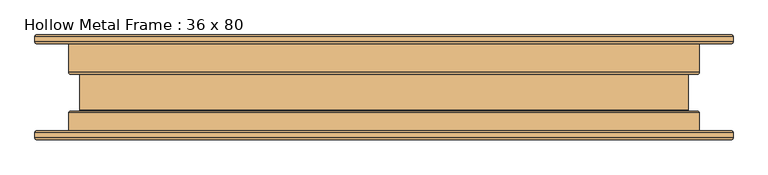
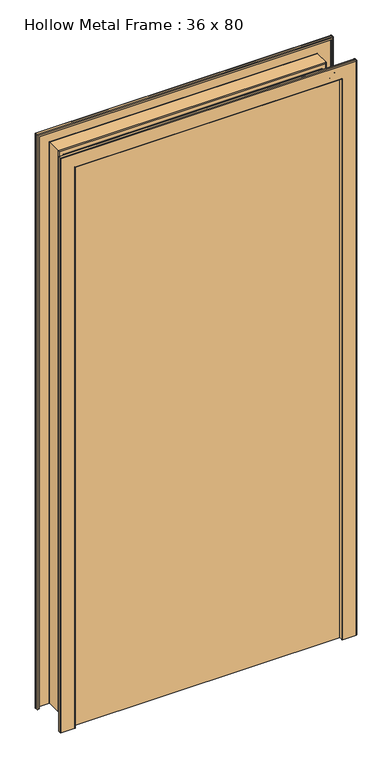
"""IFC4 building model written with IfcOpenShell, lengths in millimetres: door geometry, Hollow Metal Frame : 36 x 80."""

from ifc_helpers import new_model, si_unit, frame, origin, origin_with_axes, place, context, project, spatial, polyline, circle_curve, ellipse_curve, outline, extrude, source, transform, mapped, element, save
from ifc_brep_helpers import plane_surface, cylinder_surface, revolved_surface, advanced_brep


def hollow_metal_frame_36_x_80_d56a384a(model_context):
    return source(origin(), model_context, "Body", "SolidModel", [
        advanced_brep(
        [(-505.42825, 63.5635, 0.0), (-508.0, 66.13525, 0.0), (-508.0, 73.66, 0.0), (-505.42825, 76.23175, 0.0), (-459.77175, 76.23175, 0.0), (-457.2, 73.66, 0.0), (-457.2, 21.68525, 0.0), (-456.184, 20.66925, 0.0), (-443.89675, 20.66925, 0.0), (-441.325, 18.0975, 0.0), (-441.325, -33.6931, 0.0), (-443.89675, -36.26485, 0.0), (-456.184, -36.26485, 0.0), (-457.2, -37.28085, 0.0), (-457.2, -73.5965, 0.0), (-459.77175, -76.16825, 0.0), (-505.42825, -76.16825, 0.0), (-508.0, -73.5965, 0.0), (-508.0, -66.07175, 0.0), (-505.42825, -63.5, 0.0), (-500.0625, -63.5, 0.0), (-500.0625, -65.05575, 0.0), (-505.42825, -65.05575, 0.0), (-506.44425, -66.07175, 0.0), (-506.44425, -73.5965, 0.0), (-505.42825, -74.6125, 0.0), (-459.77175, -74.6125, 0.0), (-458.75575, -73.5965, 0.0), (-458.75575, -37.28085, 0.0), (-456.184, -34.7091, 0.0), (-443.89675, -34.7091, 0.0), (-442.88075, -33.6931, 0.0), (-442.88075, 18.0975, 0.0), (-443.89675, 19.1135, 0.0), (-456.184, 19.1135, 0.0), (-458.75575, 21.68525, 0.0), (-458.75575, 73.66, 0.0), (-459.77175, 74.676, 0.0), (-505.42825, 74.676, 0.0), (-506.44425, 73.66, 0.0), (-506.44425, 66.13525, 0.0), (-505.42825, 65.11925, 0.0), (-500.0625, 65.11925, 0.0), (-500.0625, 63.5635, 0.0), (-505.42825, 63.5635, 2080.2282501), (-508.0, 66.13525, 2082.8000001), (-508.0, 73.66, 2082.8000001), (-505.42825, 76.23175, 2080.2282501), (505.42825, 76.23175, 2080.2282501), (505.42825, 76.23175, 0.0), (459.77175, 76.23175, 0.0), (459.77175, 76.23175, 2034.5717501), (-459.77175, 76.23175, 2034.5717501), (-457.2, 73.66, 2032.0000001), (-457.2, 21.68525, 2032.0000001), (-456.184, 20.66925, 2030.9840001), (456.184, 20.66925, 2030.9840001), (456.184, 20.66925, 0.0), (443.89675, 20.66925, 0.0), (443.89675, 20.66925, 2018.6967501), (-443.89675, 20.66925, 2018.6967501), (-441.325, 18.0975, 2016.1250001), (-441.325, -33.6931, 2016.1250001), (-443.89675, -36.26485, 2018.6967501), (443.89675, -36.26485, 2018.6967501), (443.89675, -36.26485, 0.0), (456.184, -36.26485, 0.0), (456.184, -36.26485, 2030.9840001), (-456.184, -36.26485, 2030.9840001), (-457.2, -37.28085, 2032.0000001), (-457.2, -73.5965, 2032.0000001), (-459.77175, -76.16825, 2034.5717501), (459.77175, -76.16825, 2034.5717501), (459.77175, -76.16825, 0.0), (505.42825, -76.16825, 0.0), (505.42825, -76.16825, 2080.2282501), (-505.42825, -76.16825, 2080.2282501), (-508.0, -73.5965, 2082.8000001), (-508.0, -66.07175, 2082.8000001), (-505.42825, -63.5, 2080.2282501), (505.42825, -63.5, 2080.2282501), (505.42825, -63.5, 0.0), (500.0625, -63.5, 0.0), (500.0625, -63.5, 2074.8625001), (-500.0625, -63.5, 2074.8625001), (-500.0625, -65.05575, 2074.8625001), (500.0625, -65.05575, 2074.8625001), (500.0625, -65.05575, 0.0), (505.42825, -65.05575, 0.0), (505.42825, -65.05575, 2080.2282501), (-505.42825, -65.05575, 2080.2282501), (-506.44425, -66.07175, 2081.2442501), (-506.44425, -73.5965, 2081.2442501), (-505.42825, -74.6125, 2080.2282501), (505.42825, -74.6125, 2080.2282501), (505.42825, -74.6125, 0.0), (459.77175, -74.6125, 0.0), (459.77175, -74.6125, 2034.5717501), (-459.77175, -74.6125, 2034.5717501), (-458.75575, -73.5965, 2033.5557501), (-458.75575, -37.28085, 2033.5557501), (-456.184, -34.7091, 2030.9840001), (456.184, -34.7091, 2030.9840001), (456.184, -34.7091, 0.0), (443.89675, -34.7091, 0.0), (443.89675, -34.7091, 2018.6967501), (-443.89675, -34.7091, 2018.6967501), (-442.88075, -33.6931, 2017.6807501), (-442.88075, 18.0975, 2017.6807501), (-443.89675, 19.1135, 2018.6967501), (443.89675, 19.1135, 2018.6967501), (443.89675, 19.1135, 0.0), (456.184, 19.1135, 0.0), (456.184, 19.1135, 2030.9840001), (-456.184, 19.1135, 2030.9840001), (-458.75575, 21.68525, 2033.5557501), (-458.75575, 73.66, 2033.5557501), (-459.77175, 74.676, 2034.5717501), (459.77175, 74.676, 2034.5717501), (459.77175, 74.676, 0.0), (505.42825, 74.676, 0.0), (505.42825, 74.676, 2080.2282501), (-505.42825, 74.676, 2080.2282501), (-506.44425, 73.66, 2081.2442501), (-506.44425, 66.13525, 2081.2442501), (-505.42825, 65.11925, 2080.2282501), (505.42825, 65.11925, 2080.2282501), (505.42825, 65.11925, 0.0), (500.0625, 65.11925, 0.0), (500.0625, 65.11925, 2074.8625001), (-500.0625, 65.11925, 2074.8625001), (-500.0625, 63.5635, 2074.8625001), (500.0625, 63.5635, 2074.8625001), (500.0625, 63.5635, 0.0), (505.42825, 63.5635, 0.0), (505.42825, 63.5635, 2080.2282501), (508.0, 66.13525, 2082.8000001), (508.0, 73.66, 2082.8000001), (457.2, 73.66, 2032.0000001), (457.2, 21.68525, 2032.0000001), (441.325, 18.0975, 2016.1250001), (441.325, -33.6931, 2016.1250001), (457.2, -37.28085, 2032.0000001), (457.2, -73.5965, 2032.0000001), (508.0, -73.5965, 2082.8000001), (508.0, -66.07175, 2082.8000001), (506.44425, -66.07175, 2081.2442501), (506.44425, -73.5965, 2081.2442501), (458.75575, -73.5965, 2033.5557501), (458.75575, -37.28085, 2033.5557501), (442.88075, -33.6931, 2017.6807501), (442.88075, 18.0975, 2017.6807501), (458.75575, 21.68525, 2033.5557501), (458.75575, 73.66, 2033.5557501), (506.44425, 73.66, 2081.2442501), (506.44425, 66.13525, 2081.2442501), (506.44425, 66.13525, 0.0), (506.44425, 73.66, 0.0), (458.75575, 73.66, 0.0), (458.75575, 21.68525, 0.0), (442.88075, 18.0975, 0.0), (442.88075, -33.6931, 0.0), (458.75575, -37.28085, 0.0), (458.75575, -73.5965, 0.0), (506.44425, -73.5965, 0.0), (506.44425, -66.07175, 0.0), (508.0, -66.07175, 0.0), (508.0, -73.5965, 0.0), (457.2, -73.5965, 0.0), (457.2, -37.28085, 0.0), (441.325, -33.6931, 0.0), (441.325, 18.0975, 0.0), (457.2, 21.68525, 0.0), (457.2, 73.66, 0.0), (508.0, 73.66, 0.0), (508.0, 66.13525, 0.0)],
        [
            (0, 1, circle_curve(frame((-505.42825, 66.13525, 0.0), z_axis=(0.0, 0.0, -1.0), x_axis=(0.0, -1.0, 0.0)), 2.57175)),
            (1, 2),
            (2, 3, circle_curve(frame((-505.42825, 73.66, 0.0), z_axis=(0.0, 0.0, -1.0), x_axis=(0.0, -1.0, 0.0)), 2.57175)),
            (3, 4),
            (4, 5, circle_curve(frame((-459.77175, 73.66, 0.0), z_axis=(0.0, 0.0, -1.0), x_axis=(0.0, -1.0, 0.0)), 2.57175)),
            (5, 6),
            (6, 7, circle_curve(frame((-456.184, 21.68525, 0.0), z_axis=(0.0, 0.0, 1.0), x_axis=(0.0, -1.0, 0.0)), 1.016)),
            (7, 8),
            (8, 9, circle_curve(frame((-443.89675, 18.0975, 0.0), z_axis=(0.0, 0.0, -1.0), x_axis=(0.0, -1.0, 0.0)), 2.57175)),
            (9, 10),
            (10, 11, circle_curve(frame((-443.89675, -33.6931, 0.0), z_axis=(0.0, 0.0, -1.0), x_axis=(0.0, -1.0, 0.0)), 2.57175)),
            (11, 12),
            (12, 13, circle_curve(frame((-456.184, -37.28085, 0.0), z_axis=(0.0, 0.0, 1.0), x_axis=(0.0, -1.0, 0.0)), 1.016)),
            (13, 14),
            (14, 15, circle_curve(frame((-459.77175, -73.5965, 0.0), z_axis=(0.0, 0.0, -1.0), x_axis=(0.0, -1.0, 0.0)), 2.57175)),
            (15, 16),
            (16, 17, circle_curve(frame((-505.42825, -73.5965, 0.0), z_axis=(0.0, 0.0, -1.0), x_axis=(0.0, -1.0, 0.0)), 2.57175)),
            (17, 18),
            (18, 19, circle_curve(frame((-505.42825, -66.07175, 0.0), z_axis=(0.0, 0.0, -1.0), x_axis=(0.0, -1.0, 0.0)), 2.57175)),
            (19, 20),
            (20, 21),
            (21, 22),
            (22, 23, circle_curve(frame((-505.42825, -66.07175, 0.0), z_axis=(0.0, 0.0, 1.0), x_axis=(0.0, -1.0, 0.0)), 1.016)),
            (23, 24),
            (24, 25, circle_curve(frame((-505.42825, -73.5965, 0.0), z_axis=(0.0, 0.0, 1.0), x_axis=(0.0, -1.0, 0.0)), 1.016)),
            (25, 26),
            (26, 27, circle_curve(frame((-459.77175, -73.5965, 0.0), z_axis=(0.0, 0.0, 1.0), x_axis=(0.0, -1.0, 0.0)), 1.016)),
            (27, 28),
            (28, 29, circle_curve(frame((-456.184, -37.28085, 0.0), z_axis=(0.0, 0.0, -1.0), x_axis=(0.0, -1.0, 0.0)), 2.57175)),
            (29, 30),
            (30, 31, circle_curve(frame((-443.89675, -33.6931, 0.0), z_axis=(0.0, 0.0, 1.0), x_axis=(0.0, -1.0, 0.0)), 1.016)),
            (31, 32),
            (32, 33, circle_curve(frame((-443.89675, 18.0975, 0.0), z_axis=(0.0, 0.0, 1.0), x_axis=(0.0, -1.0, 0.0)), 1.016)),
            (33, 34),
            (34, 35, circle_curve(frame((-456.184, 21.68525, 0.0), z_axis=(0.0, 0.0, -1.0), x_axis=(0.0, -1.0, 0.0)), 2.57175)),
            (35, 36),
            (36, 37, circle_curve(frame((-459.77175, 73.66, 0.0), z_axis=(0.0, 0.0, 1.0), x_axis=(0.0, -1.0, 0.0)), 1.016)),
            (37, 38),
            (38, 39, circle_curve(frame((-505.42825, 73.66, 0.0), z_axis=(0.0, 0.0, 1.0), x_axis=(0.0, -1.0, 0.0)), 1.016)),
            (39, 40),
            (40, 41, circle_curve(frame((-505.42825, 66.13525, 0.0), z_axis=(0.0, 0.0, 1.0), x_axis=(0.0, -1.0, 0.0)), 1.016)),
            (41, 42),
            (42, 43),
            (43, 0),
            (0, 44),
            (44, 45, ellipse_curve(frame((-505.42825, 66.13525, 2080.2282501), z_axis=(-0.7071067811865475, 0.0, -0.7071067811865475), x_axis=(0.7071067811865474, 0.0, -0.7071067811865476)), 3.6370037, 2.57175)),
            (45, 1),
            (45, 46),
            (46, 2),
            (46, 47, ellipse_curve(frame((-505.42825, 73.66, 2080.2282501), z_axis=(-0.7071067811865475, 0.0, -0.7071067811865475), x_axis=(0.7071067811865474, 0.0, -0.7071067811865476)), 3.6370037, 2.57175)),
            (47, 3),
            (47, 48),
            (48, 49),
            (49, 50),
            (50, 51),
            (51, 52),
            (52, 4),
            (52, 53, ellipse_curve(frame((-459.77175, 73.66, 2034.5717501), z_axis=(-0.7071067811865475, 0.0, -0.7071067811865475), x_axis=(0.7071067811865474, 0.0, -0.7071067811865476)), 3.6370037, 2.57175)),
            (53, 5),
            (53, 54),
            (54, 6),
            (54, 55, ellipse_curve(frame((-456.184, 21.68525, 2030.9840001), z_axis=(0.7071067811865475, 0.0, 0.7071067811865475), x_axis=(-0.7071067811865474, 0.0, 0.7071067811865476)), 1.436841, 1.016)),
            (55, 7),
            (55, 56),
            (56, 57),
            (57, 58),
            (58, 59),
            (59, 60),
            (60, 8),
            (60, 61, ellipse_curve(frame((-443.89675, 18.0975, 2018.6967501), z_axis=(-0.7071067811865475, 0.0, -0.7071067811865475), x_axis=(0.7071067811865474, 0.0, -0.7071067811865476)), 3.6370037, 2.57175)),
            (61, 9),
            (61, 62),
            (62, 10),
            (62, 63, ellipse_curve(frame((-443.89675, -33.6931, 2018.6967501), z_axis=(-0.7071067811865475, 0.0, -0.7071067811865475), x_axis=(0.7071067811865474, 0.0, -0.7071067811865476)), 3.6370037, 2.57175)),
            (63, 11),
            (63, 64),
            (64, 65),
            (65, 66),
            (66, 67),
            (67, 68),
            (68, 12),
            (68, 69, ellipse_curve(frame((-456.184, -37.28085, 2030.9840001), z_axis=(0.7071067811865475, 0.0, 0.7071067811865475), x_axis=(-0.7071067811865474, 0.0, 0.7071067811865476)), 1.436841, 1.016)),
            (69, 13),
            (69, 70),
            (70, 14),
            (70, 71, ellipse_curve(frame((-459.77175, -73.5965, 2034.5717501), z_axis=(-0.7071067811865475, 0.0, -0.7071067811865475), x_axis=(0.7071067811865474, 0.0, -0.7071067811865476)), 3.6370037, 2.57175)),
            (71, 15),
            (71, 72),
            (72, 73),
            (73, 74),
            (74, 75),
            (75, 76),
            (76, 16),
            (76, 77, ellipse_curve(frame((-505.42825, -73.5965, 2080.2282501), z_axis=(-0.7071067811865475, 0.0, -0.7071067811865475), x_axis=(0.7071067811865474, 0.0, -0.7071067811865476)), 3.6370037, 2.57175)),
            (77, 17),
            (77, 78),
            (78, 18),
            (78, 79, ellipse_curve(frame((-505.42825, -66.07175, 2080.2282501), z_axis=(-0.7071067811865475, 0.0, -0.7071067811865475), x_axis=(0.7071067811865474, 0.0, -0.7071067811865476)), 3.6370037, 2.57175)),
            (79, 19),
            (79, 80),
            (80, 81),
            (81, 82),
            (82, 83),
            (83, 84),
            (84, 20),
            (84, 85),
            (85, 21),
            (85, 86),
            (86, 87),
            (87, 88),
            (88, 89),
            (89, 90),
            (90, 22),
            (90, 91, ellipse_curve(frame((-505.42825, -66.07175, 2080.2282501), z_axis=(0.7071067811865475, 0.0, 0.7071067811865475), x_axis=(-0.7071067811865474, 0.0, 0.7071067811865476)), 1.436841, 1.016)),
            (91, 23),
            (91, 92),
            (92, 24),
            (92, 93, ellipse_curve(frame((-505.42825, -73.5965, 2080.2282501), z_axis=(0.7071067811865475, 0.0, 0.7071067811865475), x_axis=(-0.7071067811865474, 0.0, 0.7071067811865476)), 1.436841, 1.016)),
            (93, 25),
            (93, 94),
            (94, 95),
            (95, 96),
            (96, 97),
            (97, 98),
            (98, 26),
            (98, 99, ellipse_curve(frame((-459.77175, -73.5965, 2034.5717501), z_axis=(0.7071067811865475, 0.0, 0.7071067811865475), x_axis=(-0.7071067811865474, 0.0, 0.7071067811865476)), 1.436841, 1.016)),
            (99, 27),
            (99, 100),
            (100, 28),
            (100, 101, ellipse_curve(frame((-456.184, -37.28085, 2030.9840001), z_axis=(-0.7071067811865475, 0.0, -0.7071067811865475), x_axis=(0.7071067811865474, 0.0, -0.7071067811865476)), 3.6370037, 2.57175)),
            (101, 29),
            (101, 102),
            (102, 103),
            (103, 104),
            (104, 105),
            (105, 106),
            (106, 30),
            (106, 107, ellipse_curve(frame((-443.89675, -33.6931, 2018.6967501), z_axis=(0.7071067811865475, 0.0, 0.7071067811865475), x_axis=(-0.7071067811865474, 0.0, 0.7071067811865476)), 1.436841, 1.016)),
            (107, 31),
            (107, 108),
            (108, 32),
            (108, 109, ellipse_curve(frame((-443.89675, 18.0975, 2018.6967501), z_axis=(0.7071067811865475, 0.0, 0.7071067811865475), x_axis=(-0.7071067811865474, 0.0, 0.7071067811865476)), 1.436841, 1.016)),
            (109, 33),
            (109, 110),
            (110, 111),
            (111, 112),
            (112, 113),
            (113, 114),
            (114, 34),
            (114, 115, ellipse_curve(frame((-456.184, 21.68525, 2030.9840001), z_axis=(-0.7071067811865475, 0.0, -0.7071067811865475), x_axis=(0.7071067811865474, 0.0, -0.7071067811865476)), 3.6370037, 2.57175)),
            (115, 35),
            (115, 116),
            (116, 36),
            (116, 117, ellipse_curve(frame((-459.77175, 73.66, 2034.5717501), z_axis=(0.7071067811865475, 0.0, 0.7071067811865475), x_axis=(-0.7071067811865474, 0.0, 0.7071067811865476)), 1.436841, 1.016)),
            (117, 37),
            (117, 118),
            (118, 119),
            (119, 120),
            (120, 121),
            (121, 122),
            (122, 38),
            (122, 123, ellipse_curve(frame((-505.42825, 73.66, 2080.2282501), z_axis=(0.7071067811865475, 0.0, 0.7071067811865475), x_axis=(-0.7071067811865474, 0.0, 0.7071067811865476)), 1.436841, 1.016)),
            (123, 39),
            (123, 124),
            (124, 40),
            (124, 125, ellipse_curve(frame((-505.42825, 66.13525, 2080.2282501), z_axis=(0.7071067811865475, 0.0, 0.7071067811865475), x_axis=(-0.7071067811865474, 0.0, 0.7071067811865476)), 1.436841, 1.016)),
            (125, 41),
            (125, 126),
            (126, 127),
            (127, 128),
            (128, 129),
            (129, 130),
            (130, 42),
            (130, 131),
            (131, 43),
            (131, 132),
            (132, 133),
            (133, 134),
            (134, 135),
            (135, 44),
            (135, 136, ellipse_curve(frame((505.42825, 66.13525, 2080.2282501), z_axis=(-0.7071067811865475, 0.0, 0.7071067811865475), x_axis=(-0.7071067811865476, 0.0, -0.7071067811865474)), 3.6370037, 2.57175)),
            (136, 45),
            (136, 137),
            (137, 46),
            (137, 48, ellipse_curve(frame((505.42825, 73.66, 2080.2282501), z_axis=(-0.7071067811865475, 0.0, 0.7071067811865475), x_axis=(-0.7071067811865476, 0.0, -0.7071067811865474)), 3.6370037, 2.57175)),
            (51, 138, ellipse_curve(frame((459.77175, 73.66, 2034.5717501), z_axis=(-0.7071067811865475, 0.0, 0.7071067811865475), x_axis=(-0.7071067811865476, 0.0, -0.7071067811865474)), 3.6370037, 2.57175)),
            (138, 53),
            (138, 139),
            (139, 54),
            (139, 56, ellipse_curve(frame((456.184, 21.68525, 2030.9840001), z_axis=(0.7071067811865475, 0.0, -0.7071067811865475), x_axis=(0.7071067811865476, 0.0, 0.7071067811865474)), 1.436841, 1.016)),
            (59, 140, ellipse_curve(frame((443.89675, 18.0975, 2018.6967501), z_axis=(-0.7071067811865475, 0.0, 0.7071067811865475), x_axis=(-0.7071067811865476, 0.0, -0.7071067811865474)), 3.6370037, 2.57175)),
            (140, 61),
            (140, 141),
            (141, 62),
            (141, 64, ellipse_curve(frame((443.89675, -33.6931, 2018.6967501), z_axis=(-0.7071067811865475, 0.0, 0.7071067811865475), x_axis=(-0.7071067811865476, 0.0, -0.7071067811865474)), 3.6370037, 2.57175)),
            (67, 142, ellipse_curve(frame((456.184, -37.28085, 2030.9840001), z_axis=(0.7071067811865475, 0.0, -0.7071067811865475), x_axis=(0.7071067811865476, 0.0, 0.7071067811865474)), 1.436841, 1.016)),
            (142, 69),
            (142, 143),
            (143, 70),
            (143, 72, ellipse_curve(frame((459.77175, -73.5965, 2034.5717501), z_axis=(-0.7071067811865475, 0.0, 0.7071067811865475), x_axis=(-0.7071067811865476, 0.0, -0.7071067811865474)), 3.6370037, 2.57175)),
            (75, 144, ellipse_curve(frame((505.42825, -73.5965, 2080.2282501), z_axis=(-0.7071067811865475, 0.0, 0.7071067811865475), x_axis=(-0.7071067811865476, 0.0, -0.7071067811865474)), 3.6370037, 2.57175)),
            (144, 77),
            (144, 145),
            (145, 78),
            (145, 80, ellipse_curve(frame((505.42825, -66.07175, 2080.2282501), z_axis=(-0.7071067811865475, 0.0, 0.7071067811865475), x_axis=(-0.7071067811865476, 0.0, -0.7071067811865474)), 3.6370037, 2.57175)),
            (83, 86),
            (89, 146, ellipse_curve(frame((505.42825, -66.07175, 2080.2282501), z_axis=(0.7071067811865475, 0.0, -0.7071067811865475), x_axis=(0.7071067811865476, 0.0, 0.7071067811865474)), 1.436841, 1.016)),
            (146, 91),
            (146, 147),
            (147, 92),
            (147, 94, ellipse_curve(frame((505.42825, -73.5965, 2080.2282501), z_axis=(0.7071067811865475, 0.0, -0.7071067811865475), x_axis=(0.7071067811865476, 0.0, 0.7071067811865474)), 1.436841, 1.016)),
            (97, 148, ellipse_curve(frame((459.77175, -73.5965, 2034.5717501), z_axis=(0.7071067811865475, 0.0, -0.7071067811865475), x_axis=(0.7071067811865476, 0.0, 0.7071067811865474)), 1.436841, 1.016)),
            (148, 99),
            (148, 149),
            (149, 100),
            (149, 102, ellipse_curve(frame((456.184, -37.28085, 2030.9840001), z_axis=(-0.7071067811865475, 0.0, 0.7071067811865475), x_axis=(-0.7071067811865476, 0.0, -0.7071067811865474)), 3.6370037, 2.57175)),
            (105, 150, ellipse_curve(frame((443.89675, -33.6931, 2018.6967501), z_axis=(0.7071067811865475, 0.0, -0.7071067811865475), x_axis=(0.7071067811865476, 0.0, 0.7071067811865474)), 1.436841, 1.016)),
            (150, 107),
            (150, 151),
            (151, 108),
            (151, 110, ellipse_curve(frame((443.89675, 18.0975, 2018.6967501), z_axis=(0.7071067811865475, 0.0, -0.7071067811865475), x_axis=(0.7071067811865476, 0.0, 0.7071067811865474)), 1.436841, 1.016)),
            (113, 152, ellipse_curve(frame((456.184, 21.68525, 2030.9840001), z_axis=(-0.7071067811865475, 0.0, 0.7071067811865475), x_axis=(-0.7071067811865476, 0.0, -0.7071067811865474)), 3.6370037, 2.57175)),
            (152, 115),
            (152, 153),
            (153, 116),
            (153, 118, ellipse_curve(frame((459.77175, 73.66, 2034.5717501), z_axis=(0.7071067811865475, 0.0, -0.7071067811865475), x_axis=(0.7071067811865476, 0.0, 0.7071067811865474)), 1.436841, 1.016)),
            (121, 154, ellipse_curve(frame((505.42825, 73.66, 2080.2282501), z_axis=(0.7071067811865475, 0.0, -0.7071067811865475), x_axis=(0.7071067811865476, 0.0, 0.7071067811865474)), 1.436841, 1.016)),
            (154, 123),
            (154, 155),
            (155, 124),
            (155, 126, ellipse_curve(frame((505.42825, 66.13525, 2080.2282501), z_axis=(0.7071067811865475, 0.0, -0.7071067811865475), x_axis=(0.7071067811865476, 0.0, 0.7071067811865474)), 1.436841, 1.016)),
            (129, 132),
            (133, 128),
            (127, 156, circle_curve(frame((505.42825, 66.13525, 0.0), z_axis=(0.0, 0.0, 1.0), x_axis=(0.0, -1.0, 0.0)), 1.016)),
            (156, 157),
            (157, 120, circle_curve(frame((505.42825, 73.66, 0.0), z_axis=(0.0, 0.0, 1.0), x_axis=(0.0, -1.0, 0.0)), 1.016)),
            (119, 158, circle_curve(frame((459.77175, 73.66, 0.0), z_axis=(0.0, 0.0, 1.0), x_axis=(0.0, -1.0, 0.0)), 1.016)),
            (158, 159),
            (159, 112, circle_curve(frame((456.184, 21.68525, 0.0), z_axis=(0.0, 0.0, -1.0), x_axis=(0.0, -1.0, 0.0)), 2.57175)),
            (111, 160, circle_curve(frame((443.89675, 18.0975, 0.0), z_axis=(0.0, 0.0, 1.0), x_axis=(0.0, -1.0, 0.0)), 1.016)),
            (160, 161),
            (161, 104, circle_curve(frame((443.89675, -33.6931, 0.0), z_axis=(0.0, 0.0, 1.0), x_axis=(0.0, -1.0, 0.0)), 1.016)),
            (103, 162, circle_curve(frame((456.184, -37.28085, 0.0), z_axis=(0.0, 0.0, -1.0), x_axis=(0.0, -1.0, 0.0)), 2.57175)),
            (162, 163),
            (163, 96, circle_curve(frame((459.77175, -73.5965, 0.0), z_axis=(0.0, 0.0, 1.0), x_axis=(0.0, -1.0, 0.0)), 1.016)),
            (95, 164, circle_curve(frame((505.42825, -73.5965, 0.0), z_axis=(0.0, 0.0, 1.0), x_axis=(0.0, -1.0, 0.0)), 1.016)),
            (164, 165),
            (165, 88, circle_curve(frame((505.42825, -66.07175, 0.0), z_axis=(0.0, 0.0, 1.0), x_axis=(0.0, -1.0, 0.0)), 1.016)),
            (87, 82),
            (81, 166, circle_curve(frame((505.42825, -66.07175, 0.0), z_axis=(0.0, 0.0, -1.0), x_axis=(0.0, -1.0, 0.0)), 2.57175)),
            (166, 167),
            (167, 74, circle_curve(frame((505.42825, -73.5965, 0.0), z_axis=(0.0, 0.0, -1.0), x_axis=(0.0, -1.0, 0.0)), 2.57175)),
            (73, 168, circle_curve(frame((459.77175, -73.5965, 0.0), z_axis=(0.0, 0.0, -1.0), x_axis=(0.0, -1.0, 0.0)), 2.57175)),
            (168, 169),
            (169, 66, circle_curve(frame((456.184, -37.28085, 0.0), z_axis=(0.0, 0.0, 1.0), x_axis=(0.0, -1.0, 0.0)), 1.016)),
            (65, 170, circle_curve(frame((443.89675, -33.6931, 0.0), z_axis=(0.0, 0.0, -1.0), x_axis=(0.0, -1.0, 0.0)), 2.57175)),
            (170, 171),
            (171, 58, circle_curve(frame((443.89675, 18.0975, 0.0), z_axis=(0.0, 0.0, -1.0), x_axis=(0.0, -1.0, 0.0)), 2.57175)),
            (57, 172, circle_curve(frame((456.184, 21.68525, 0.0), z_axis=(0.0, 0.0, 1.0), x_axis=(0.0, -1.0, 0.0)), 1.016)),
            (172, 173),
            (173, 50, circle_curve(frame((459.77175, 73.66, 0.0), z_axis=(0.0, 0.0, -1.0), x_axis=(0.0, -1.0, 0.0)), 2.57175)),
            (49, 174, circle_curve(frame((505.42825, 73.66, 0.0), z_axis=(0.0, 0.0, -1.0), x_axis=(0.0, -1.0, 0.0)), 2.57175)),
            (174, 175),
            (175, 134, circle_curve(frame((505.42825, 66.13525, 0.0), z_axis=(0.0, 0.0, -1.0), x_axis=(0.0, -1.0, 0.0)), 2.57175)),
            (175, 136),
            (174, 137),
            (173, 138),
            (172, 139),
            (171, 140),
            (170, 141),
            (169, 142),
            (168, 143),
            (167, 144),
            (166, 145),
            (165, 146),
            (164, 147),
            (163, 148),
            (162, 149),
            (161, 150),
            (160, 151),
            (159, 152),
            (158, 153),
            (157, 154),
            (156, 155),
        ],
        [
            plane_surface(frame((-468.3125, -63.5, 0.0), z_axis=(0.0, 0.0, -1.0), x_axis=(1.0, 0.0, 0.0))),
            cylinder_surface(frame((-505.42825, 66.13525, 0.0), z_axis=(0.0, 0.0, -1.0), x_axis=(0.0, -1.0, 0.0)), 2.57175),
            plane_surface(frame((-508.0, 66.13525, 0.0), z_axis=(-1.0, 0.0, 0.0), x_axis=(0.0, 0.0, 1.0))),
            cylinder_surface(frame((-505.42825, 73.66, 0.0), z_axis=(0.0, 0.0, -1.0), x_axis=(0.0, -1.0, 0.0)), 2.57175),
            plane_surface(frame((-505.42825, 76.23175, 0.0), z_axis=(0.0, 1.0, 0.0), x_axis=(0.0, 0.0, 1.0))),
            cylinder_surface(frame((-459.77175, 73.66, 0.0), z_axis=(0.0, 0.0, -1.0), x_axis=(0.0, -1.0, 0.0)), 2.57175),
            plane_surface(frame((-457.2, 73.66, 0.0), z_axis=(1.0, 0.0, 0.0), x_axis=(0.0, 0.0, 1.0))),
            revolved_surface(polyline([(-456.184, 20.669249999999998, 2032.0000001145868), (-456.184, 20.669249999999998, 0.0)]), (-456.184, 21.68525, 0.0), (0.0, 0.0, 1.0)),
            plane_surface(frame((-456.184, 20.66925, 0.0), z_axis=(0.0, 1.0, 0.0), x_axis=(0.0, 0.0, 1.0))),
            cylinder_surface(frame((-443.89675, 18.0975, 0.0), z_axis=(0.0, 0.0, -1.0), x_axis=(0.0, -1.0, 0.0)), 2.57175),
            plane_surface(frame((-441.325, 18.0975, 0.0), z_axis=(1.0, 0.0, 0.0), x_axis=(0.0, 0.0, 1.0))),
            cylinder_surface(frame((-443.89675, -33.6931, 0.0), z_axis=(0.0, 0.0, -1.0), x_axis=(0.0, -1.0, 0.0)), 2.57175),
            plane_surface(frame((-443.89675, -36.26485, 0.0), z_axis=(0.0, -1.0, 0.0), x_axis=(0.0, 0.0, 1.0))),
            revolved_surface(polyline([(-456.184, -38.29685, 2032.0000001145868), (-456.184, -38.29685, 0.0)]), (-456.184, -37.28085, 0.0), (0.0, 0.0, 1.0)),
            plane_surface(frame((-457.2, -37.28085, 0.0), z_axis=(1.0, 0.0, 0.0), x_axis=(0.0, 0.0, 1.0))),
            cylinder_surface(frame((-459.77175, -73.5965, 0.0), z_axis=(0.0, 0.0, -1.0), x_axis=(0.0, -1.0, 0.0)), 2.57175),
            plane_surface(frame((-459.77175, -76.16825, 0.0), z_axis=(0.0, -1.0, 0.0), x_axis=(0.0, 0.0, 1.0))),
            cylinder_surface(frame((-505.42825, -73.5965, 0.0), z_axis=(0.0, 0.0, -1.0), x_axis=(0.0, -1.0, 0.0)), 2.57175),
            plane_surface(frame((-508.0, -73.5965, 0.0), z_axis=(-1.0, 0.0, 0.0), x_axis=(0.0, 0.0, 1.0))),
            cylinder_surface(frame((-505.42825, -66.07175, 0.0), z_axis=(0.0, 0.0, -1.0), x_axis=(0.0, -1.0, 0.0)), 2.57175),
            plane_surface(frame((-505.42825, -63.5, 0.0), z_axis=(0.0, 1.0, 0.0), x_axis=(0.0, 0.0, 1.0))),
            plane_surface(frame((-500.0625, -63.5, 0.0), z_axis=(1.0, 0.0, 0.0), x_axis=(0.0, 0.0, 1.0))),
            plane_surface(frame((-500.0625, -65.05575, 0.0), z_axis=(0.0, -1.0, 0.0), x_axis=(0.0, 0.0, 1.0))),
            revolved_surface(polyline([(-505.42825, -67.08775, 2081.244250114587), (-505.42825, -67.08775, 0.0)]), (-505.42825, -66.07175, 0.0), (0.0, 0.0, 1.0)),
            plane_surface(frame((-506.44425, -66.07175, 0.0), z_axis=(1.0, 0.0, 0.0), x_axis=(0.0, 0.0, 1.0))),
            revolved_surface(polyline([(-505.42825, -74.61250000000001, 2081.244250114587), (-505.42825, -74.61250000000001, 0.0)]), (-505.42825, -73.5965, 0.0), (0.0, 0.0, 1.0)),
            plane_surface(frame((-505.42825, -74.6125, 0.0), z_axis=(0.0, 1.0, 0.0), x_axis=(0.0, 0.0, 1.0))),
            revolved_surface(polyline([(-459.77175, -74.61250000000001, 2035.5877501145867), (-459.77175, -74.61250000000001, 0.0)]), (-459.77175, -73.5965, 0.0), (0.0, 0.0, 1.0)),
            plane_surface(frame((-458.75575, -73.5965, 0.0), z_axis=(-1.0, 0.0, 0.0), x_axis=(0.0, 0.0, 1.0))),
            cylinder_surface(frame((-456.184, -37.28085, 0.0), z_axis=(0.0, 0.0, -1.0), x_axis=(0.0, -1.0, 0.0)), 2.57175),
            plane_surface(frame((-456.184, -34.7091, 0.0), z_axis=(0.0, 1.0, 0.0), x_axis=(0.0, 0.0, 1.0))),
            revolved_surface(polyline([(-443.89675, -34.7091, 2019.7127501145867), (-443.89675, -34.7091, 0.0)]), (-443.89675, -33.6931, 0.0), (0.0, 0.0, 1.0)),
            plane_surface(frame((-442.88075, -33.6931, 0.0), z_axis=(-1.0, 0.0, 0.0), x_axis=(0.0, 0.0, 1.0))),
            revolved_surface(polyline([(-443.89675, 17.0815, 2019.7127501145867), (-443.89675, 17.0815, 0.0)]), (-443.89675, 18.0975, 0.0), (0.0, 0.0, 1.0)),
            plane_surface(frame((-443.89675, 19.1135, 0.0), z_axis=(0.0, -1.0, 0.0), x_axis=(0.0, 0.0, 1.0))),
            cylinder_surface(frame((-456.184, 21.68525, 0.0), z_axis=(0.0, 0.0, -1.0), x_axis=(0.0, -1.0, 0.0)), 2.57175),
            plane_surface(frame((-458.75575, 21.68525, 0.0), z_axis=(-1.0, 0.0, 0.0), x_axis=(0.0, 0.0, 1.0))),
            revolved_surface(polyline([(-459.77175, 72.64399999999999, 2035.5877501145867), (-459.77175, 72.64399999999999, 0.0)]), (-459.77175, 73.66, 0.0), (0.0, 0.0, 1.0)),
            plane_surface(frame((-459.77175, 74.676, 0.0), z_axis=(0.0, -1.0, 0.0), x_axis=(0.0, 0.0, 1.0))),
            revolved_surface(polyline([(-505.42825, 72.64399999999999, 2081.244250114587), (-505.42825, 72.64399999999999, 0.0)]), (-505.42825, 73.66, 0.0), (0.0, 0.0, 1.0)),
            plane_surface(frame((-506.44425, 73.66, 0.0), z_axis=(1.0, 0.0, 0.0), x_axis=(0.0, 0.0, 1.0))),
            revolved_surface(polyline([(-505.42825, 65.11925, 2081.244250114587), (-505.42825, 65.11925, 0.0)]), (-505.42825, 66.13525, 0.0), (0.0, 0.0, 1.0)),
            plane_surface(frame((-505.42825, 65.11925, 0.0), z_axis=(0.0, 1.0, 0.0), x_axis=(0.0, 0.0, 1.0))),
            plane_surface(frame((-500.0625, 65.11925, 0.0), z_axis=(1.0, 0.0, 0.0), x_axis=(0.0, 0.0, 1.0))),
            plane_surface(frame((-500.0625, 63.5635, 0.0), z_axis=(0.0, -1.0, 0.0), x_axis=(0.0, 0.0, 1.0))),
            cylinder_surface(frame((-468.3125, 66.13525, 2080.2282501), z_axis=(-1.0, 0.0, 0.0), x_axis=(0.0, -1.0, 0.0)), 2.57175),
            plane_surface(frame((-508.0, 66.13525, 2082.8000001), z_axis=(0.0, 0.0, 1.0), x_axis=(1.0, 0.0, 0.0))),
            cylinder_surface(frame((-468.3125, 73.66, 2080.2282501), z_axis=(-1.0, 0.0, 0.0), x_axis=(0.0, -1.0, 0.0)), 2.57175),
            cylinder_surface(frame((-468.3125, 73.66, 2034.5717501), z_axis=(-1.0, 0.0, 0.0), x_axis=(0.0, -1.0, 0.0)), 2.57175),
            plane_surface(frame((-457.2, 73.66, 2032.0000001), z_axis=(0.0, 0.0, -1.0), x_axis=(1.0, 0.0, 0.0))),
            revolved_surface(polyline([(457.20000001458686, 20.669249999999998, 2030.9840001), (-457.20000001458686, 20.669249999999998, 2030.9840001)]), (-468.3125, 21.68525, 2030.9840001), (1.0, 0.0, 0.0)),
            cylinder_surface(frame((-468.3125, 18.0975, 2018.6967501), z_axis=(-1.0, 0.0, 0.0), x_axis=(0.0, -1.0, 0.0)), 2.57175),
            plane_surface(frame((-441.325, 18.0975, 2016.1250001), z_axis=(0.0, 0.0, -1.0), x_axis=(1.0, 0.0, 0.0))),
            cylinder_surface(frame((-468.3125, -33.6931, 2018.6967501), z_axis=(-1.0, 0.0, 0.0), x_axis=(0.0, -1.0, 0.0)), 2.57175),
            revolved_surface(polyline([(457.20000001458686, -38.29685, 2030.9840001), (-457.20000001458686, -38.29685, 2030.9840001)]), (-468.3125, -37.28085, 2030.9840001), (1.0, 0.0, 0.0)),
            plane_surface(frame((-457.2, -37.28085, 2032.0000001), z_axis=(0.0, 0.0, -1.0), x_axis=(1.0, 0.0, 0.0))),
            cylinder_surface(frame((-468.3125, -73.5965, 2034.5717501), z_axis=(-1.0, 0.0, 0.0), x_axis=(0.0, -1.0, 0.0)), 2.57175),
            cylinder_surface(frame((-468.3125, -73.5965, 2080.2282501), z_axis=(-1.0, 0.0, 0.0), x_axis=(0.0, -1.0, 0.0)), 2.57175),
            plane_surface(frame((-508.0, -73.5965, 2082.8000001), z_axis=(0.0, 0.0, 1.0), x_axis=(1.0, 0.0, 0.0))),
            cylinder_surface(frame((-468.3125, -66.07175, 2080.2282501), z_axis=(-1.0, 0.0, 0.0), x_axis=(0.0, -1.0, 0.0)), 2.57175),
            plane_surface(frame((-500.0625, -63.5, 2074.8625001), z_axis=(0.0, 0.0, -1.0), x_axis=(1.0, 0.0, 0.0))),
            revolved_surface(polyline([(506.4442500145868, -67.08775, 2080.2282501), (-506.4442500145868, -67.08775, 2080.2282501)]), (-468.3125, -66.07175, 2080.2282501), (1.0, 0.0, 0.0)),
            plane_surface(frame((-506.44425, -66.07175, 2081.2442501), z_axis=(0.0, 0.0, -1.0), x_axis=(1.0, 0.0, 0.0))),
            revolved_surface(polyline([(506.4442500145868, -74.61250000000001, 2080.2282501), (-506.4442500145868, -74.61250000000001, 2080.2282501)]), (-468.3125, -73.5965, 2080.2282501), (1.0, 0.0, 0.0)),
            revolved_surface(polyline([(460.7877500145869, -74.61250000000001, 2034.5717501), (-460.78775001458683, -74.61250000000001, 2034.5717501)]), (-468.3125, -73.5965, 2034.5717501), (1.0, 0.0, 0.0)),
            plane_surface(frame((-458.75575, -73.5965, 2033.5557501), z_axis=(0.0, 0.0, 1.0), x_axis=(1.0, 0.0, 0.0))),
            cylinder_surface(frame((-468.3125, -37.28085, 2030.9840001), z_axis=(-1.0, 0.0, 0.0), x_axis=(0.0, -1.0, 0.0)), 2.57175),
            revolved_surface(polyline([(444.9127500145869, -34.7091, 2018.6967501), (-444.91275001458683, -34.7091, 2018.6967501)]), (-468.3125, -33.6931, 2018.6967501), (1.0, 0.0, 0.0)),
            plane_surface(frame((-442.88075, -33.6931, 2017.6807501), z_axis=(0.0, 0.0, 1.0), x_axis=(1.0, 0.0, 0.0))),
            revolved_surface(polyline([(444.9127500145869, 17.0815, 2018.6967501), (-444.91275001458683, 17.0815, 2018.6967501)]), (-468.3125, 18.0975, 2018.6967501), (1.0, 0.0, 0.0)),
            cylinder_surface(frame((-468.3125, 21.68525, 2030.9840001), z_axis=(-1.0, 0.0, 0.0), x_axis=(0.0, -1.0, 0.0)), 2.57175),
            plane_surface(frame((-458.75575, 21.68525, 2033.5557501), z_axis=(0.0, 0.0, 1.0), x_axis=(1.0, 0.0, 0.0))),
            revolved_surface(polyline([(460.7877500145869, 72.64399999999999, 2034.5717501), (-460.78775001458683, 72.64399999999999, 2034.5717501)]), (-468.3125, 73.66, 2034.5717501), (1.0, 0.0, 0.0)),
            revolved_surface(polyline([(506.4442500145868, 72.64399999999999, 2080.2282501), (-506.4442500145868, 72.64399999999999, 2080.2282501)]), (-468.3125, 73.66, 2080.2282501), (1.0, 0.0, 0.0)),
            plane_surface(frame((-506.44425, 73.66, 2081.2442501), z_axis=(0.0, 0.0, -1.0), x_axis=(1.0, 0.0, 0.0))),
            revolved_surface(polyline([(506.4442500145868, 65.11925, 2080.2282501), (-506.4442500145868, 65.11925, 2080.2282501)]), (-468.3125, 66.13525, 2080.2282501), (1.0, 0.0, 0.0)),
            plane_surface(frame((-500.0625, 65.11925, 2074.8625001), z_axis=(0.0, 0.0, -1.0), x_axis=(1.0, 0.0, 0.0))),
            plane_surface(frame((468.3125, -63.5, 0.0), z_axis=(0.0, 0.0, -1.0), x_axis=(-1.0, 0.0, 0.0))),
            cylinder_surface(frame((505.42825, 66.13525, 2043.1125001), z_axis=(0.0, 0.0, 1.0), x_axis=(0.0, -1.0, 0.0)), 2.57175),
            plane_surface(frame((508.0, 66.13525, 2082.8000001), z_axis=(1.0, 0.0, 0.0), x_axis=(0.0, 0.0, -1.0))),
            cylinder_surface(frame((505.42825, 73.66, 2043.1125001), z_axis=(0.0, 0.0, 1.0), x_axis=(0.0, -1.0, 0.0)), 2.57175),
            cylinder_surface(frame((459.77175, 73.66, 2043.1125001), z_axis=(0.0, 0.0, 1.0), x_axis=(0.0, -1.0, 0.0)), 2.57175),
            plane_surface(frame((457.2, 73.66, 2032.0000001), z_axis=(-1.0, 0.0, 0.0), x_axis=(0.0, 0.0, -1.0))),
            revolved_surface(polyline([(456.184, 20.669249999999998, 0.0), (456.184, 20.669249999999998, 2032.0000001145868)]), (456.184, 21.68525, 2043.1125001), (0.0, 0.0, -1.0)),
            cylinder_surface(frame((443.89675, 18.0975, 2043.1125001), z_axis=(0.0, 0.0, 1.0), x_axis=(0.0, -1.0, 0.0)), 2.57175),
            plane_surface(frame((441.325, 18.0975, 2016.1250001), z_axis=(-1.0, 0.0, 0.0), x_axis=(0.0, 0.0, -1.0))),
            cylinder_surface(frame((443.89675, -33.6931, 2043.1125001), z_axis=(0.0, 0.0, 1.0), x_axis=(0.0, -1.0, 0.0)), 2.57175),
            revolved_surface(polyline([(456.184, -38.29685, 0.0), (456.184, -38.29685, 2032.0000001145868)]), (456.184, -37.28085, 2043.1125001), (0.0, 0.0, -1.0)),
            plane_surface(frame((457.2, -37.28085, 2032.0000001), z_axis=(-1.0, 0.0, 0.0), x_axis=(0.0, 0.0, -1.0))),
            cylinder_surface(frame((459.77175, -73.5965, 2043.1125001), z_axis=(0.0, 0.0, 1.0), x_axis=(0.0, -1.0, 0.0)), 2.57175),
            cylinder_surface(frame((505.42825, -73.5965, 2043.1125001), z_axis=(0.0, 0.0, 1.0), x_axis=(0.0, -1.0, 0.0)), 2.57175),
            plane_surface(frame((508.0, -73.5965, 2082.8000001), z_axis=(1.0, 0.0, 0.0), x_axis=(0.0, 0.0, -1.0))),
            cylinder_surface(frame((505.42825, -66.07175, 2043.1125001), z_axis=(0.0, 0.0, 1.0), x_axis=(0.0, -1.0, 0.0)), 2.57175),
            plane_surface(frame((500.0625, -63.5, 2074.8625001), z_axis=(-1.0, 0.0, 0.0), x_axis=(0.0, 0.0, -1.0))),
            revolved_surface(polyline([(505.42825, -67.08775, 0.0), (505.42825, -67.08775, 2081.244250114587)]), (505.42825, -66.07175, 2043.1125001), (0.0, 0.0, -1.0)),
            plane_surface(frame((506.44425, -66.07175, 2081.2442501), z_axis=(-1.0, 0.0, 0.0), x_axis=(0.0, 0.0, -1.0))),
            revolved_surface(polyline([(505.42825, -74.61250000000001, 0.0), (505.42825, -74.61250000000001, 2081.244250114587)]), (505.42825, -73.5965, 2043.1125001), (0.0, 0.0, -1.0)),
            revolved_surface(polyline([(459.77175, -74.61250000000001, 0.0), (459.77175, -74.61250000000001, 2035.5877501145867)]), (459.77175, -73.5965, 2043.1125001), (0.0, 0.0, -1.0)),
            plane_surface(frame((458.75575, -73.5965, 2033.5557501), z_axis=(1.0, 0.0, 0.0), x_axis=(0.0, 0.0, -1.0))),
            cylinder_surface(frame((456.184, -37.28085, 2043.1125001), z_axis=(0.0, 0.0, 1.0), x_axis=(0.0, -1.0, 0.0)), 2.57175),
            revolved_surface(polyline([(443.89675, -34.7091, 0.0), (443.89675, -34.7091, 2019.7127501145867)]), (443.89675, -33.6931, 2043.1125001), (0.0, 0.0, -1.0)),
            plane_surface(frame((442.88075, -33.6931, 2017.6807501), z_axis=(1.0, 0.0, 0.0), x_axis=(0.0, 0.0, -1.0))),
            revolved_surface(polyline([(443.89675, 17.0815, 0.0), (443.89675, 17.0815, 2019.7127501145867)]), (443.89675, 18.0975, 2043.1125001), (0.0, 0.0, -1.0)),
            cylinder_surface(frame((456.184, 21.68525, 2043.1125001), z_axis=(0.0, 0.0, 1.0), x_axis=(0.0, -1.0, 0.0)), 2.57175),
            plane_surface(frame((458.75575, 21.68525, 2033.5557501), z_axis=(1.0, 0.0, 0.0), x_axis=(0.0, 0.0, -1.0))),
            revolved_surface(polyline([(459.77175, 72.64399999999999, 0.0), (459.77175, 72.64399999999999, 2035.5877501145867)]), (459.77175, 73.66, 2043.1125001), (0.0, 0.0, -1.0)),
            revolved_surface(polyline([(505.42825, 72.64399999999999, 0.0), (505.42825, 72.64399999999999, 2081.244250114587)]), (505.42825, 73.66, 2043.1125001), (0.0, 0.0, -1.0)),
            plane_surface(frame((506.44425, 73.66, 2081.2442501), z_axis=(-1.0, 0.0, 0.0), x_axis=(0.0, 0.0, -1.0))),
            revolved_surface(polyline([(505.42825, 65.11925, 0.0), (505.42825, 65.11925, 2081.244250114587)]), (505.42825, 66.13525, 2043.1125001), (0.0, 0.0, -1.0)),
            plane_surface(frame((500.0625, 65.11925, 2074.8625001), z_axis=(-1.0, 0.0, 0.0), x_axis=(0.0, 0.0, -1.0))),
        ],
        [
            (0, [[1, 2, 3, 4, 5, 6, 7, 8, 9, 10, 11, 12, 13, 14, 15, 16, 17, 18, 19, 20, 21, 22, 23, 24, 25, 26, 27, 28, 29, 30, 31, 32, 33, 34, 35, 36, 37, 38, 39, 40, 41, 42, 43, 44]]),
            (1, [[-1, 45, 46, 47]]),
            (2, [[-2, -47, 48, 49]]),
            (3, [[-3, -49, 50, 51]]),
            (4, [[-4, -51, 52, 53, 54, 55, 56, 57]]),
            (5, [[-5, -57, 58, 59]]),
            (6, [[-6, -59, 60, 61]]),
            (7, [[-7, -61, 62, 63]]),
            (8, [[-8, -63, 64, 65, 66, 67, 68, 69]]),
            (9, [[-9, -69, 70, 71]]),
            (10, [[-10, -71, 72, 73]]),
            (11, [[-11, -73, 74, 75]]),
            (12, [[-12, -75, 76, 77, 78, 79, 80, 81]]),
            (13, [[-13, -81, 82, 83]]),
            (14, [[-14, -83, 84, 85]]),
            (15, [[-15, -85, 86, 87]]),
            (16, [[-16, -87, 88, 89, 90, 91, 92, 93]]),
            (17, [[-17, -93, 94, 95]]),
            (18, [[-18, -95, 96, 97]]),
            (19, [[-19, -97, 98, 99]]),
            (20, [[-20, -99, 100, 101, 102, 103, 104, 105]]),
            (21, [[-21, -105, 106, 107]]),
            (22, [[-22, -107, 108, 109, 110, 111, 112, 113]]),
            (23, [[-23, -113, 114, 115]]),
            (24, [[-24, -115, 116, 117]]),
            (25, [[-25, -117, 118, 119]]),
            (26, [[-26, -119, 120, 121, 122, 123, 124, 125]]),
            (27, [[-27, -125, 126, 127]]),
            (28, [[-28, -127, 128, 129]]),
            (29, [[-29, -129, 130, 131]]),
            (30, [[-30, -131, 132, 133, 134, 135, 136, 137]]),
            (31, [[-31, -137, 138, 139]]),
            (32, [[-32, -139, 140, 141]]),
            (33, [[-33, -141, 142, 143]]),
            (34, [[-34, -143, 144, 145, 146, 147, 148, 149]]),
            (35, [[-35, -149, 150, 151]]),
            (36, [[-36, -151, 152, 153]]),
            (37, [[-37, -153, 154, 155]]),
            (38, [[-38, -155, 156, 157, 158, 159, 160, 161]]),
            (39, [[-39, -161, 162, 163]]),
            (40, [[-40, -163, 164, 165]]),
            (41, [[-41, -165, 166, 167]]),
            (42, [[-42, -167, 168, 169, 170, 171, 172, 173]]),
            (43, [[-43, -173, 174, 175]]),
            (44, [[-44, -175, 176, 177, 178, 179, 180, -45]]),
            (45, [[-46, -180, 181, 182]]),
            (46, [[-48, -182, 183, 184]]),
            (47, [[-50, -184, 185, -52]]),
            (48, [[-58, -56, 186, 187]]),
            (49, [[-60, -187, 188, 189]]),
            (50, [[-62, -189, 190, -64]]),
            (51, [[-70, -68, 191, 192]]),
            (52, [[-72, -192, 193, 194]]),
            (53, [[-74, -194, 195, -76]]),
            (54, [[-82, -80, 196, 197]]),
            (55, [[-84, -197, 198, 199]]),
            (56, [[-86, -199, 200, -88]]),
            (57, [[-94, -92, 201, 202]]),
            (58, [[-96, -202, 203, 204]]),
            (59, [[-98, -204, 205, -100]]),
            (60, [[-106, -104, 206, -108]]),
            (61, [[-114, -112, 207, 208]]),
            (62, [[-116, -208, 209, 210]]),
            (63, [[-118, -210, 211, -120]]),
            (64, [[-126, -124, 212, 213]]),
            (65, [[-128, -213, 214, 215]]),
            (66, [[-130, -215, 216, -132]]),
            (67, [[-138, -136, 217, 218]]),
            (68, [[-140, -218, 219, 220]]),
            (69, [[-142, -220, 221, -144]]),
            (70, [[-150, -148, 222, 223]]),
            (71, [[-152, -223, 224, 225]]),
            (72, [[-154, -225, 226, -156]]),
            (73, [[-162, -160, 227, 228]]),
            (74, [[-164, -228, 229, 230]]),
            (75, [[-166, -230, 231, -168]]),
            (76, [[-174, -172, 232, -176]]),
            (77, [[-178, 233, -170, 234, 235, 236, -158, 237, 238, 239, -146, 240, 241, 242, -134, 243, 244, 245, -122, 246, 247, 248, -110, 249, -102, 250, 251, 252, -90, 253, 254, 255, -78, 256, 257, 258, -66, 259, 260, 261, -54, 262, 263, 264]]),
            (78, [[-181, -179, -264, 265]]),
            (79, [[-183, -265, -263, 266]]),
            (80, [[-185, -266, -262, -53]]),
            (81, [[-186, -55, -261, 267]]),
            (82, [[-188, -267, -260, 268]]),
            (83, [[-190, -268, -259, -65]]),
            (84, [[-191, -67, -258, 269]]),
            (85, [[-193, -269, -257, 270]]),
            (86, [[-195, -270, -256, -77]]),
            (87, [[-196, -79, -255, 271]]),
            (88, [[-198, -271, -254, 272]]),
            (89, [[-200, -272, -253, -89]]),
            (90, [[-201, -91, -252, 273]]),
            (91, [[-203, -273, -251, 274]]),
            (92, [[-205, -274, -250, -101]]),
            (93, [[-206, -103, -249, -109]]),
            (94, [[-207, -111, -248, 275]]),
            (95, [[-209, -275, -247, 276]]),
            (96, [[-211, -276, -246, -121]]),
            (97, [[-212, -123, -245, 277]]),
            (98, [[-214, -277, -244, 278]]),
            (99, [[-216, -278, -243, -133]]),
            (100, [[-217, -135, -242, 279]]),
            (101, [[-219, -279, -241, 280]]),
            (102, [[-221, -280, -240, -145]]),
            (103, [[-222, -147, -239, 281]]),
            (104, [[-224, -281, -238, 282]]),
            (105, [[-226, -282, -237, -157]]),
            (106, [[-227, -159, -236, 283]]),
            (107, [[-229, -283, -235, 284]]),
            (108, [[-231, -284, -234, -169]]),
            (109, [[-232, -171, -233, -177]]),
        ],
    ),
        extrude(outline(polyline([(455.64425, -37.28085), (455.64425, -63.5), (-455.64425, -63.5), (-455.64425, -37.28085), (455.64425, -37.28085)])), origin_with_axes(), (0.0, 0.0, 1.0), 2032.0000001),
    ])


if __name__ == "__main__":
    model = new_model("IFC4")
    model_context = context("Model", 3, world=origin())
    ifc_project = project(units=[si_unit("LENGTHUNIT", "METRE", prefix="MILLI")], contexts=[model_context])
    site = spatial("IfcSite", under=ifc_project)
    building = spatial("IfcBuilding", under=site)
    placement = place(None, origin())
    hollow_metal_frame_36_x_80_shape = hollow_metal_frame_36_x_80_d56a384a(model_context)
    element("IfcDoor", 1, ObjectType="Hollow Metal Frame : 36 x 80", at=placement, inside=building, context=model_context, shape_type="MappedRepresentation", body=[
        mapped(hollow_metal_frame_36_x_80_shape, transform((0.0, 0.0, 0.0), x_axis=(1.0, 0.0, 0.0), y_axis=(0.0, 1.0, 0.0), z_axis=(0.0, 0.0, 1.0))),
    ])
    save(model, "model.ifc")

# Revit data of these elements
# Type "Hollow Metal Frame : 36 x 80"
#   Type Mark = "g"
#   Product Page URL = ""
#   Product Name = ""
#   Product Documentation Link = ""
#   Material = ""
#   DS_Hardware_Set_(SFT) = ""
#   DS_Frame_Type_(SFT) = ""
#   DS_Fire_Rating_(SFT) = ""
#   DS_Door_Type_(SFT) = ""
#   Analytic Construction = "<None>"
#   Frame Projection Ext. = 0' - 1"
#   Frame Projection Int. = 0' - 1"
#   Frame Width = 0' - 3"
#   Height = 6' - 8"
#   Width = 3' - 0"
#   Non-Kerfed = yes
#   Kerfed = no
#   Hollow Metal Casing = Metal-Dunbarton_Doors-White
#   Flush Door = Metal-Dunbarton_Doors-Aluminum
#   DS_Frame_Material_(SFT) = none
#   DS_Door_Material_(SFT) = none
#   URL = ""
#   Model = ""
#   Manufacturer = ""
#   Function = (empty or 0)
#   Wall Closure = (empty or 0)
#   Description = (empty or 0)
# Element 1 (IfcDoor, "Hollow Metal Frame : 36 x 80")
#   Materials on its faces: "Metal-Dunbarton_Doors-White", "Metal-Dunbarton_Doors-Aluminum"
# Materials
#   "Metal-Dunbarton_Doors-White": class "Miscellaneous", colour RGB 230 233 236, transparency 0
#   "Metal-Dunbarton_Doors-Aluminum": class "System", colour RGB 143 142 141, transparency 0
